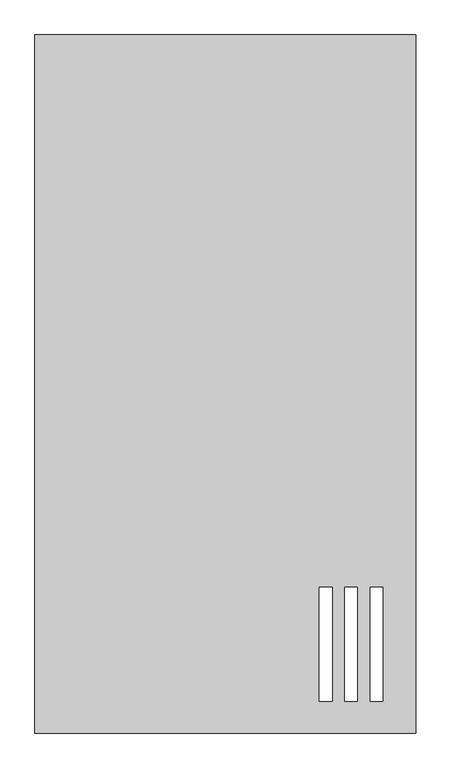
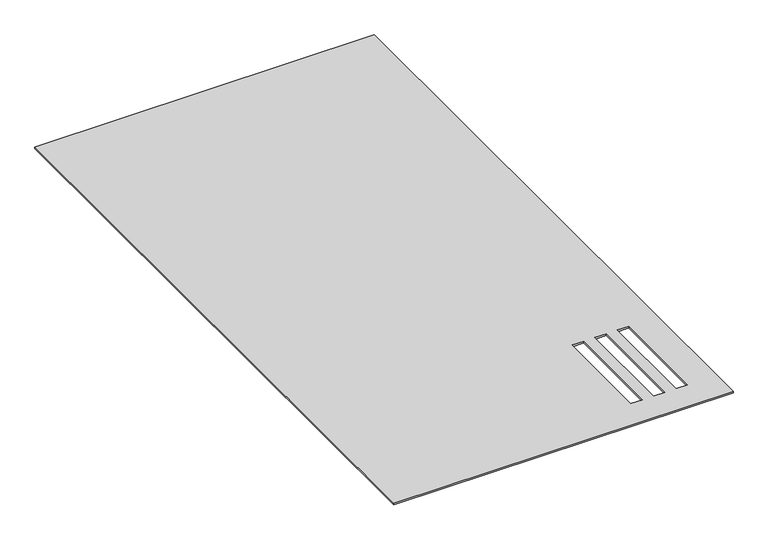
"""IFC4 building model written with IfcOpenShell, lengths in millimetres: proxy geometry, TSP Geyser Solar 300L : TSP Geyser Solar 300L."""

from ifc_helpers import new_model, si_unit, origin, origin_with_axes, place, context, project, spatial, polyline, outline, extrude, source, transform, mapped, element, save


def electrical_fixtures_5c64e13b(model_context):
    return source(origin(), model_context, "Body", "SweptSolid", [
        extrude(outline(polyline([(-600.0, 600.0), (0.0, 600.0), (0.0, -500.0), (-600.0, -500.0), (-600.0, 600.0)]), holes=[polyline([(-71.8082825, -450.0), (-51.8082825, -450.0), (-51.8082825, -270.0), (-71.8082825, -270.0), (-71.8082825, -450.0)]), polyline([(-111.8082825, -450.0), (-91.8082825, -450.0), (-91.8082825, -270.0), (-111.8082825, -270.0), (-111.8082825, -450.0)]), polyline([(-151.8082825, -450.0), (-131.8082825, -450.0), (-131.8082825, -270.0), (-151.8082825, -270.0), (-151.8082825, -450.0)])]), origin_with_axes(), (0.0, 0.0, 1.0), 3.0),
    ])


if __name__ == "__main__":
    model = new_model("IFC4")
    model_context = context("Model", 3, world=origin())
    ifc_project = project(units=[si_unit("LENGTHUNIT", "METRE", prefix="MILLI")], contexts=[model_context])
    site = spatial("IfcSite", under=ifc_project)
    building = spatial("IfcBuilding", under=site)
    placement = place(None, origin())
    electrical_fixtures_shape = electrical_fixtures_5c64e13b(model_context)
    element("IfcBuildingElementProxy", 1, Name="TSP Geyser Solar 300L : TSP Geyser Solar 300L", ObjectType="TSP Geyser Solar 300L : TSP Geyser Solar 300L", at=placement, inside=building, context=model_context, shape_type="MappedRepresentation", body=[
        mapped(electrical_fixtures_shape, transform((0.0, 0.0, 0.0), x_axis=(1.0, 0.0, 0.0), y_axis=(0.0, 1.0, 0.0), z_axis=(0.0, 0.0, 1.0))),
    ])
    save(model, "model.ifc")

# Revit data of these elements
# Type "TSP Geyser Solar 300L : TSP Geyser Solar 300L"
#   Model = "TSP_SGEY300"
#   Default Elevation = 0
# Element 1 (IfcBuildingElementProxy, "TSP Geyser Solar 300L : TSP Geyser Solar 300L")
#   Materials on its faces: "Aluminum, Anodized Red"
# Materials
#   "Aluminum, Anodized Red": class "Metal", colour RGB 120 120 120, transparency 0, Description = "Anodized aluminum, red", Cost = 0
